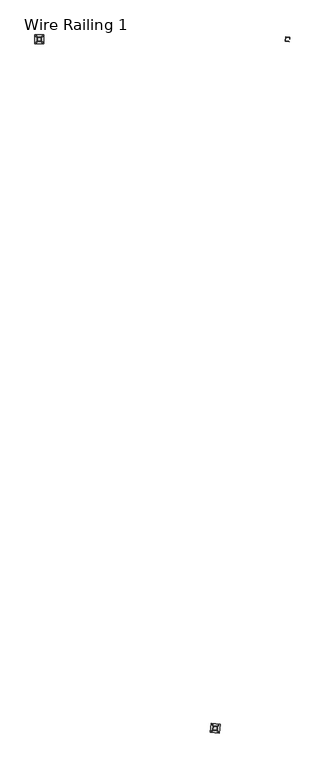
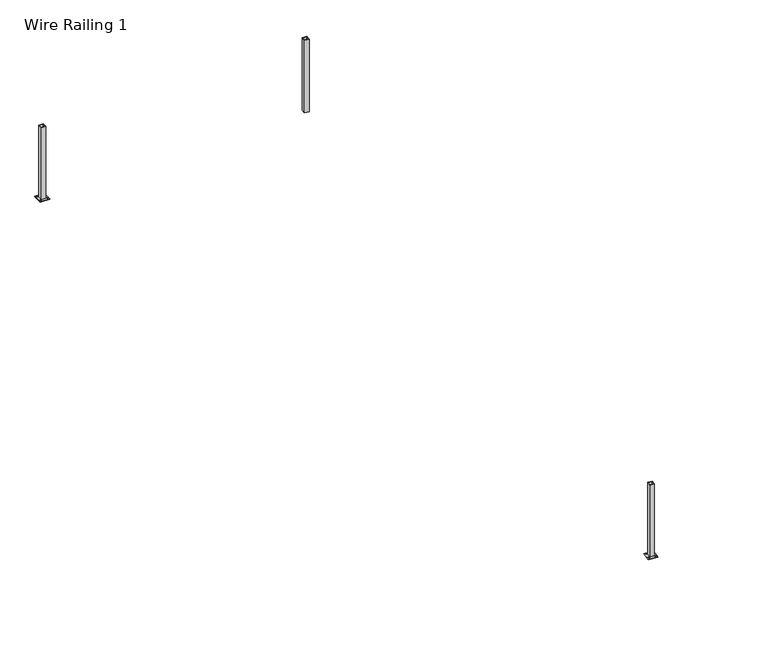
"""IFC4 building model written with IfcOpenShell, lengths in millimetres: railing geometry, Wire Railing 1."""

from ifc_helpers import new_model, si_unit, point, frame, frame_2d, origin, place, context, project, spatial, polyline, circle_curve, trimmed, segment, composite_curve, outline, extrude, source, transform, mapped, element, save


def wire_railing_1_b18b4590(model_context):
    return source(origin(), model_context, "Body", "SweptSolid", [
        extrude(outline(polyline([(35354.857147, 40834.1980548), (35294.8626137, 40840.5037343), (35301.1682932, 40900.4982676), (35361.1628266, 40894.1925881), (35354.857147, 40834.1980548)]), holes=[polyline([(35349.2056887, 40841.1770245), (35354.1838568, 40888.5411298), (35306.8197515, 40893.5192979), (35301.8415835, 40846.1551926), (35349.2056887, 40841.1770245)])]), frame((0.0, 0.0, 269252.7), z_axis=(0.0, 0.0, 1.0), x_axis=(1.0, 0.0, 0.0)), (0.0, 0.0, 1.0), 1047.75),
        extrude(outline(composite_curve([segment(trimmed(circle_curve(frame_2d((31766.8284681, 40822.8981612)), 6.35), [point((31766.8284681, 40816.5481612))], [point((31766.8284681, 40829.2481612))], False, "CARTESIAN"), True, "CONTINUOUS"), segment(trimmed(circle_curve(frame_2d((31766.8284681, 40822.8981612)), 6.35), [point((31766.8284681, 40829.2481612))], [point((31766.8284681, 40816.5481612))], False, "CARTESIAN"), True, "CONTINUOUS")], self_intersect=False)), frame((0.0, 0.0, 269252.7), z_axis=(0.0, 0.0, 1.0), x_axis=(1.0, 0.0, 0.0)), (0.0, 0.0, 1.0), 12.7),
        extrude(outline(composite_curve([segment(trimmed(circle_curve(frame_2d((31766.8284681, 40911.7981612)), 6.35), [point((31766.8284681, 40905.4481612))], [point((31766.8284681, 40918.1481612))], False, "CARTESIAN"), True, "CONTINUOUS"), segment(trimmed(circle_curve(frame_2d((31766.8284681, 40911.7981612)), 6.35), [point((31766.8284681, 40918.1481612))], [point((31766.8284681, 40905.4481612))], False, "CARTESIAN"), True, "CONTINUOUS")], self_intersect=False)), frame((0.0, 0.0, 269252.7), z_axis=(0.0, 0.0, 1.0), x_axis=(1.0, 0.0, 0.0)), (0.0, 0.0, 1.0), 12.7),
        extrude(outline(composite_curve([segment(trimmed(circle_curve(frame_2d((31677.9284681, 40822.8981612)), 6.35), [point((31677.9284681, 40816.5481612))], [point((31677.9284681, 40829.2481612))], False, "CARTESIAN"), True, "CONTINUOUS"), segment(trimmed(circle_curve(frame_2d((31677.9284681, 40822.8981612)), 6.35), [point((31677.9284681, 40829.2481612))], [point((31677.9284681, 40816.5481612))], False, "CARTESIAN"), True, "CONTINUOUS")], self_intersect=False)), frame((0.0, 0.0, 269252.7), z_axis=(0.0, 0.0, 1.0), x_axis=(1.0, 0.0, 0.0)), (0.0, 0.0, 1.0), 12.7),
        extrude(outline(composite_curve([segment(trimmed(circle_curve(frame_2d((31677.9284681, 40911.7981612)), 6.35), [point((31677.9284681, 40905.4481612))], [point((31677.9284681, 40918.1481612))], False, "CARTESIAN"), True, "CONTINUOUS"), segment(trimmed(circle_curve(frame_2d((31677.9284681, 40911.7981612)), 6.35), [point((31677.9284681, 40918.1481612))], [point((31677.9284681, 40905.4481612))], False, "CARTESIAN"), True, "CONTINUOUS")], self_intersect=False)), frame((0.0, 0.0, 269252.7), z_axis=(0.0, 0.0, 1.0), x_axis=(1.0, 0.0, 0.0)), (0.0, 0.0, 1.0), 12.7),
        extrude(outline(polyline([(31785.8784681, 40930.8481612), (31785.8784681, 40803.8481612), (31658.8784681, 40803.8481612), (31658.8784681, 40930.8481612), (31785.8784681, 40930.8481612)])), frame((0.0, 0.0, 269252.7), z_axis=(0.0, 0.0, 1.0), x_axis=(1.0, 0.0, 0.0)), (0.0, 0.0, 1.0), 6.35),
        extrude(outline(polyline([(31752.5409681, 40897.5106612), (31752.5409681, 40837.1856612), (31692.2159681, 40837.1856612), (31692.2159681, 40897.5106612), (31752.5409681, 40897.5106612)]), holes=[polyline([(31746.1909681, 40891.1606612), (31698.5659681, 40891.1606612), (31698.5659681, 40843.5356612), (31746.1909681, 40843.5356612), (31746.1909681, 40891.1606612)])]), frame((0.0, 0.0, 269252.7), z_axis=(0.0, 0.0, 1.0), x_axis=(1.0, 0.0, 0.0)), (0.0, 0.0, 1.0), 1047.75),
        extrude(outline(composite_curve([segment(trimmed(circle_curve(frame_2d((34227.7211326, 30824.0160171)), 6.35), [point((34221.4059185, 30824.6797728))], [point((34234.0363466, 30823.3522613))], False, "CARTESIAN"), True, "CONTINUOUS"), segment(trimmed(circle_curve(frame_2d((34227.7211326, 30824.0160171)), 6.35), [point((34234.0363466, 30823.3522613))], [point((34221.4059185, 30824.6797728))], False, "CARTESIAN"), True, "CONTINUOUS")], self_intersect=False)), frame((0.0, 0.0, 269252.7), z_axis=(0.0, 0.0, 1.0), x_axis=(1.0, 0.0, 0.0)), (0.0, 0.0, 1.0), 12.7),
        extrude(outline(composite_curve([segment(trimmed(circle_curve(frame_2d((34316.1341291, 30814.7234367)), 6.35), [point((34309.818915, 30815.3871924))], [point((34322.4493431, 30814.0596809))], False, "CARTESIAN"), True, "CONTINUOUS"), segment(trimmed(circle_curve(frame_2d((34316.1341291, 30814.7234367)), 6.35), [point((34322.4493431, 30814.0596809))], [point((34309.818915, 30815.3871924))], False, "CARTESIAN"), True, "CONTINUOUS")], self_intersect=False)), frame((0.0, 0.0, 269252.7), z_axis=(0.0, 0.0, 1.0), x_axis=(1.0, 0.0, 0.0)), (0.0, 0.0, 1.0), 12.7),
        extrude(outline(composite_curve([segment(trimmed(circle_curve(frame_2d((34237.013713, 30912.4290136)), 6.35), [point((34230.6984989, 30913.0927693))], [point((34243.328927, 30911.7652578))], False, "CARTESIAN"), True, "CONTINUOUS"), segment(trimmed(circle_curve(frame_2d((34237.013713, 30912.4290136)), 6.35), [point((34243.328927, 30911.7652578))], [point((34230.6984989, 30913.0927693))], False, "CARTESIAN"), True, "CONTINUOUS")], self_intersect=False)), frame((0.0, 0.0, 269252.7), z_axis=(0.0, 0.0, 1.0), x_axis=(1.0, 0.0, 0.0)), (0.0, 0.0, 1.0), 12.7),
        extrude(outline(composite_curve([segment(trimmed(circle_curve(frame_2d((34325.4267095, 30903.1364332)), 6.35), [point((34319.1114954, 30903.8001889))], [point((34331.7419235, 30902.4726774))], False, "CARTESIAN"), True, "CONTINUOUS"), segment(trimmed(circle_curve(frame_2d((34325.4267095, 30903.1364332)), 6.35), [point((34331.7419235, 30902.4726774))], [point((34319.1114954, 30903.8001889))], False, "CARTESIAN"), True, "CONTINUOUS")], self_intersect=False)), frame((0.0, 0.0, 269252.7), z_axis=(0.0, 0.0, 1.0), x_axis=(1.0, 0.0, 0.0)), (0.0, 0.0, 1.0), 12.7),
        extrude(outline(polyline([(34333.088504, 30793.7865273), (34206.7842232, 30807.0616422), (34220.0593381, 30933.3659229), (34346.3636188, 30920.0908081), (34333.088504, 30793.7865273)])), frame((0.0, 0.0, 269252.7), z_axis=(0.0, 0.0, 1.0), x_axis=(1.0, 0.0, 0.0)), (0.0, 0.0, 1.0), 6.35),
        extrude(outline(polyline([(34303.4183479, 30830.4261187), (34243.4238146, 30836.7317982), (34249.7294941, 30896.7263316), (34309.7240275, 30890.420652), (34303.4183479, 30830.4261187)]), holes=[polyline([(34297.7668896, 30837.4050885), (34302.7450577, 30884.7691937), (34255.3809524, 30889.7473618), (34250.4027844, 30842.3832565), (34297.7668896, 30837.4050885)])]), frame((0.0, 0.0, 269252.7), z_axis=(0.0, 0.0, 1.0), x_axis=(1.0, 0.0, 0.0)), (0.0, 0.0, 1.0), 1047.75),
    ])


if __name__ == "__main__":
    model = new_model("IFC4")
    model_context = context("Model", 3, world=origin())
    ifc_project = project(units=[si_unit("LENGTHUNIT", "METRE", prefix="MILLI")], contexts=[model_context])
    site = spatial("IfcSite", under=ifc_project)
    building = spatial("IfcBuilding", under=site)
    placement = place(None, origin())
    wire_railing_1_shape = wire_railing_1_b18b4590(model_context)
    element("IfcRailing", 1, ObjectType="Wire Railing 1", at=placement, inside=building, context=model_context, shape_type="MappedRepresentation", body=[
        mapped(wire_railing_1_shape, transform((0.0, 0.0, 0.0), x_axis=(1.0, 0.0, 0.0), y_axis=(0.0, 1.0, 0.0), z_axis=(0.0, 0.0, 1.0))),
    ])
    save(model, "model.ifc")

# Revit data of these elements
# Element 1 (IfcRailing, "Wire Railing 1")
#   Materials on its faces: "WIRE RAILING"
# Materials
#   "WIRE RAILING": class "Metal", colour RGB 244 244 244, transparency 0, Manufacturer = "Kawneer", URL = "http://www.kawneer.com/kawneer/north_america/en/home.asp", Cost = 0
